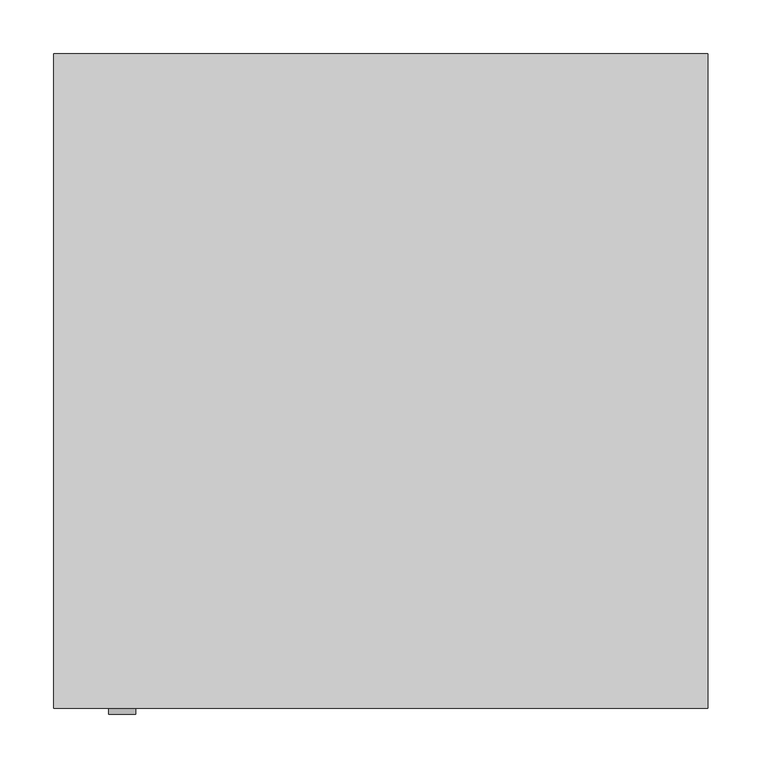
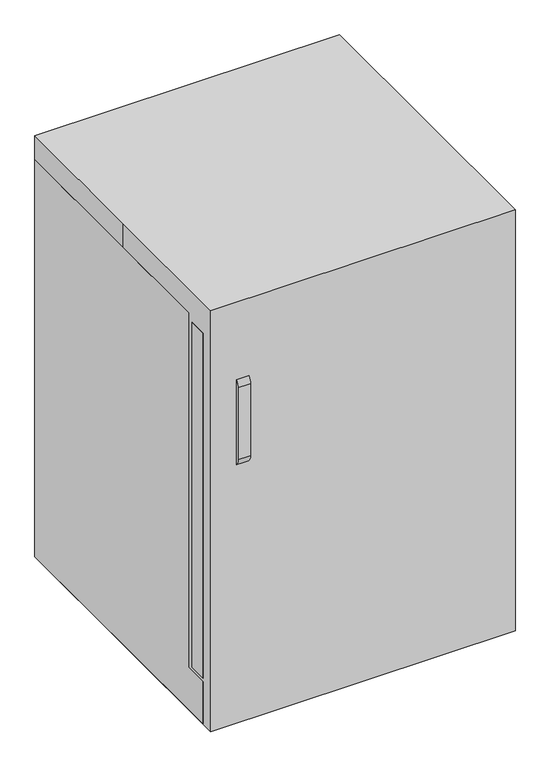
"""IFC4 building model written with IfcOpenShell, lengths in millimetres: proxy geometry, R5135 - Freezer, Undercounter, 5 Cubic Feet : R5135 - Freezer, Undercounter, 5 Cubic Feet."""

from ifc_helpers import new_model, si_unit, point, frame, frame_2d, origin, origin_with_axes, place, context, project, spatial, polyline, circle_curve, trimmed, segment, composite_curve, outline, extrude, source, transform, mapped, element, save


def specialty_equipment_3c4c7319(model_context):
    return source(origin(), model_context, "Body", "SweptSolid", [
        extrude(outline(polyline([(304.8, -278.4731993), (232.0741382, -278.4731993), (232.0741382, -227.6731993), (304.8, -227.6731993), (304.8, -278.4731993)])), frame((0.0, 0.0, 825.5), z_axis=(0.0, 0.0, 1.0), x_axis=(1.0, 0.0, 0.0)), (0.0, 0.0, 1.0), 12.7),
        extrude(outline(composite_curve([segment(polyline([(-278.4731993, 546.4738531), (-278.4731993, 540.1238531), (-291.1731993, 540.1238531)]), True, "CONTINUOUS"), segment(trimmed(circle_curve(frame_2d((-291.1731993, 559.1738531)), 19.05), [point((-291.1731993, 540.1238531))], [point((-310.2231993, 559.1738531))], False, "CARTESIAN"), True, "CONTINUOUS"), segment(polyline([(-310.2231993, 559.1738531), (-310.2231993, 711.5738531)]), True, "CONTINUOUS"), segment(trimmed(circle_curve(frame_2d((-291.1731993, 711.5738531)), 19.05), [point((-310.2231993, 711.5738531))], [point((-291.1731993, 730.6238531))], False, "CARTESIAN"), True, "CONTINUOUS"), segment(polyline([(-291.1731993, 730.6238531), (-278.4731993, 730.6238531), (-278.4731993, 724.2738531), (-291.1731993, 724.2738531)]), True, "CONTINUOUS"), segment(trimmed(circle_curve(frame_2d((-291.1731993, 711.5738531)), 12.7), [point((-291.1731993, 724.2738531))], [point((-303.8731993, 711.5738531))], True, "CARTESIAN"), True, "CONTINUOUS"), segment(polyline([(-303.8731993, 711.5738531), (-303.8731993, 559.1738531)]), True, "CONTINUOUS"), segment(trimmed(circle_curve(frame_2d((-291.1731993, 559.1738531)), 12.7), [point((-303.8731993, 559.1738531))], [point((-291.1731993, 546.4738531))], True, "CARTESIAN"), True, "CONTINUOUS"), segment(polyline([(-291.1731993, 546.4738531), (-278.4731993, 546.4738531)]), True, "CONTINUOUS")], self_intersect=False)), frame((-253.6261469, 0.0, 0.0), z_axis=(1.0, 0.0, 0.0), x_axis=(0.0, 1.0, 0.0)), (0.0, 0.0, 1.0), 25.4),
        extrude(outline(polyline([(304.8, -278.4731993), (-304.8, -278.4731993), (-304.8, -240.3731993), (304.8, -240.3731993), (304.8, -278.4731993)])), frame((0.0, 0.0, 96.7063414), z_axis=(0.0, 0.0, 1.0), x_axis=(1.0, 0.0, 0.0)), (0.0, 0.0, 1.0), 728.7936586),
        extrude(outline(polyline([(292.1, -227.6731993), (292.1, -240.3731993), (-292.4220728, -240.3731993), (-292.4220728, -227.6731993), (292.1, -227.6731993)])), frame((0.0, 0.0, 117.3428444), z_axis=(0.0, 0.0, 1.0), x_axis=(1.0, 0.0, 0.0)), (0.0, 0.0, 1.0), 691.4472963),
        extrude(outline(polyline([(-227.6731993, 838.2), (26.3268007, 838.2), (304.8, 838.2), (304.8, 0.0), (-227.6731993, 0.0), (-278.4731993, 0.0), (-278.4731993, 88.9), (-227.6731993, 88.9), (-227.6731993, 838.2)])), frame((-304.8, 0.0, 0.0), z_axis=(1.0, 0.0, 0.0), x_axis=(0.0, 1.0, 0.0)), (0.0, 0.0, 1.0), 609.6),
        extrude(outline(polyline([(-304.8, 304.8), (304.8, 304.8), (304.8, -304.8), (-304.8, -304.8), (-304.8, 0.0), (-304.8, 304.8)])), origin_with_axes(), (0.0, 0.0, 1.0), 889.0),
    ])


if __name__ == "__main__":
    model = new_model("IFC4")
    model_context = context("Model", 3, world=origin())
    ifc_project = project(units=[si_unit("LENGTHUNIT", "METRE", prefix="MILLI")], contexts=[model_context])
    site = spatial("IfcSite", under=ifc_project)
    building = spatial("IfcBuilding", under=site)
    placement = place(None, origin())
    specialty_equipment_shape = specialty_equipment_3c4c7319(model_context)
    element("IfcBuildingElementProxy", 1, Name="R5135 - Freezer, Undercounter, 5 Cubic Feet : R5135 - Freezer, Undercounter, 5 Cubic Feet", ObjectType="R5135 - Freezer, Undercounter, 5 Cubic Feet : R5135 - Freezer, Undercounter, 5 Cubic Feet", at=placement, inside=building, context=model_context, shape_type="MappedRepresentation", body=[
        mapped(specialty_equipment_shape, transform((0.0, 0.0, 0.0), x_axis=(1.0, 0.0, 0.0), y_axis=(0.0, 1.0, 0.0), z_axis=(0.0, 0.0, 1.0))),
    ])
    save(model, "model.ifc")

# Revit data of these elements
# Project information
#   Room Abbreviation = "PTTC1"
#   Room Description = "Treatment Cubicle, Physical Therapy (PTTC1)"
#   Sheets - Total = "5"
#   Project Issue Date = "Issue Date"
#   Project Status = "Project Status"
#   Client Name = "Owner"
#   Project Address = "Enter address here"
#   Project Name = "Project Name"
#   Project Number = "Project Number"
#   Publication Date = "30-Jan-15"
# Type "R5135 - Freezer, Undercounter, 5 Cubic Feet : R5135 - Freezer, Undercounter, 5 Cubic Feet"
#   Watts2 = "0"
#   Watts1 = "720"
#   Unit_Issue = "EA"
#   UTIL_6_Misc = "-"
#   UTIL_5_NonMedGas = "-"
#   UTIL_4_MiscGas = "-"
#   UTIL_3_MedGas = "-"
#   UTIL_2_Elec = "A"
#   UTIL_1_WaterDrain = "-"
#   Nomenclature = "Freezer, Undercounter, 5 Cubic Feet"
#   NSN = "4110"
#   Location [instance default] = ""
#   JSN = "R5135"
#   Fund_Source_VA = "-"
#   Fund_Source_Navy = "-"
#   Fund_Source_Army = "-"
#   Fund_Source_AF = "-"
#   ELEC_Volts2 = "0"
#   ELEC_Volts1 = "120"
#   ELEC_Phase2 = "0"
#   ELEC_Phase1 = "1"
#   ELEC_HertzSwitch = "0"
#   ELEC_HertzDependent = "-1"
#   ELEC_Hertz = "60"
#   ELEC_Amps2 = "0"
#   ELEC_Amps1 = "6"
#   DetailDescription = "Under counter freezer. This unit features space-saving thin-wall construction and has the flexibility of being built with existing cabinets, installed under-counter without top or custom-finished to specifications. This unit is a general purpose laboratory freezer."
#   CAT_VA = "C"
#   CAT_Navy = "C"
#   CAT_IHS = "-"
#   CAT_Army = "C"
#   CAT_AF = "C"
#   BTUperhour = "0"
#   Weight_IP = 190
#   DIM_Width_IP = 2' - 0"
#   DIM_Height_IP = 2' - 11"
#   DIM_Depth_IP = 2' - 0"
# Element 1 (IfcBuildingElementProxy, "R5135 - Freezer, Undercounter, 5 Cubic Feet : R5135 - Freezer, Undercounter, 5 Cubic Feet")
#   Materials on its faces: "EquipSpace"
# Materials
#   "EquipSpace": class "Unassigned", colour RGB 221 217 195, transparency 0.5
